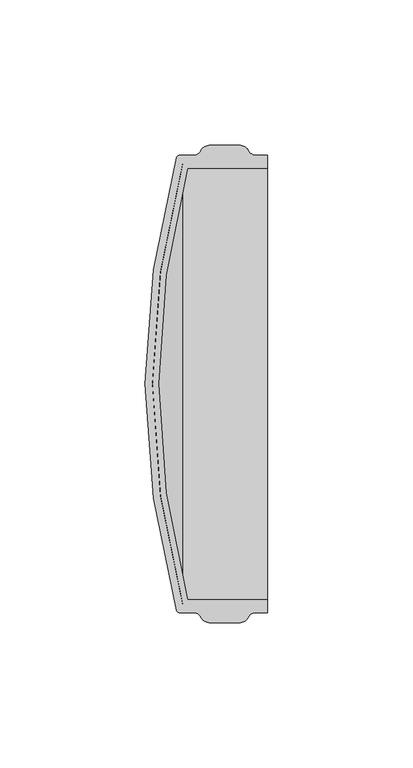
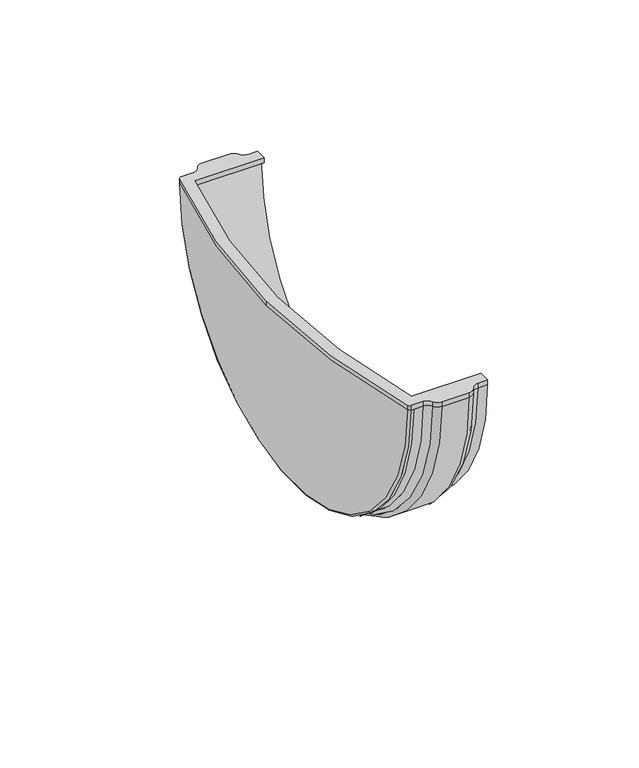
"""IFC4 building model written with IfcOpenShell, lengths in millimetres: proxy geometry, ↩ Заглушка желоба : ↩ Заглушка желоба."""

from ifc_helpers import new_model, si_unit, point, frame, origin, place, context, project, spatial, polyline, circle_curve, ellipse_curve, trimmed, source, transform, mapped, element, save
from ifc_brep_helpers import plane_surface, cylinder_surface, revolved_surface, advanced_brep


def generic_models_4d5a007a(model_context):
    return source(origin(), model_context, "Body", "AdvancedBrep", [
        advanced_brep(
        [(-25.5074023, 78.6, 0.0), (-25.5074023, -78.6, 0.0), (-29.0, -78.6, 0.0), (-29.0, 78.6, 0.0), (-22.8037012, 80.3, 0.0), (-22.8037012, -80.3, 0.0), (-20.1, 82.0, 0.0), (-20.1, -82.0, 0.0), (-9.3443413, 82.0, 0.0), (-9.3443413, -82.0, 0.0), (-6.6406401, 80.3, 0.0), (-6.6406401, -80.3, 0.0), (-3.936939, 78.6, 0.0), (-3.936939, -78.6, 0.0), (-0.0443413, 78.6, 0.0), (-0.0443413, -78.6, 0.0), (-0.0443413, 78.6, 2.0), (-0.0443413, 74.1, 2.0), (-0.0443413, 74.1, 0.0), (-0.0443413, 76.1, 0.0), (-0.0443413, -76.1, 0.0), (-0.0443413, -74.1, 0.0), (-0.0443413, -74.1, 2.0), (-0.0443413, -78.6, 2.0), (-29.0, 76.1, 0.0), (-29.0, -76.1, 0.0), (-31.2572877, 77.8330313, 0.0), (-31.2572877, -77.8330313, 0.0), (-42.0295138, 0.0, 0.0), (-30.2504109, 78.6, 0.0), (-30.2504109, -78.6, 0.0), (-39.5258282, 0.0, 0.0), (-3.936939, 78.6, 2.0), (-6.6406401, 80.3, 2.0), (-9.3443413, 82.0, 2.0), (-20.1, 82.0, 2.0), (-22.8037012, 80.3, 2.0), (-25.5074023, 78.6, 2.0), (-30.2504109, 78.6, 2.0), (-31.2572877, 77.8330313, 2.0), (-42.0295138, 0.0, 2.0), (-31.2572877, -77.8330313, 2.0), (-30.2504109, -78.6, 2.0), (-25.5074023, -78.6, 2.0), (-22.8037012, -80.3, 2.0), (-20.1, -82.0, 2.0), (-9.3443413, -82.0, 2.0), (-6.6406401, -80.3, 2.0), (-3.936939, -78.6, 2.0), (-27.4693868, -74.1, 2.0), (-37.5257643, 0.0, 2.0), (-27.4693868, 74.1, 2.0), (-27.4693868, 74.1, 0.0), (-37.5257643, 0.0, 0.0), (-27.4693868, -74.1, 0.0)],
        [
            (0, 1, circle_curve(frame((-25.5074023, 0.0, 0.0), z_axis=(-1.0, 0.0, 0.0), x_axis=(0.0, -1.0, 0.0)), 78.6)),
            (1, 2),
            (2, 3, circle_curve(frame((-29.0, 0.0, 0.0), z_axis=(1.0, 0.0, 0.0), x_axis=(0.0, -1.0, 0.0)), 78.6)),
            (3, 0),
            (0, 4, circle_curve(frame((-25.5074023, 81.6, 0.0), z_axis=(0.0, 0.0, 1.0), x_axis=(1.0, 0.0, 0.0)), 3.0)),
            (4, 5, circle_curve(frame((-22.8037012, 0.0, 0.0), z_axis=(-1.0, 0.0, 0.0), x_axis=(0.0, -1.0, 0.0)), 80.3)),
            (5, 1, circle_curve(frame((-25.5074023, -81.6, 0.0), z_axis=(0.0, 0.0, 1.0), x_axis=(1.0, 0.0, 0.0)), 3.0)),
            (4, 6, circle_curve(frame((-20.1, 79.0, 0.0), z_axis=(0.0, 0.0, -1.0), x_axis=(1.0, 0.0, 0.0)), 3.0)),
            (6, 7, circle_curve(frame((-20.1, 0.0, 0.0), z_axis=(-1.0, 0.0, 0.0), x_axis=(0.0, -1.0, 0.0)), 82.0)),
            (7, 5, circle_curve(frame((-20.1, -79.0, 0.0), z_axis=(0.0, 0.0, -1.0), x_axis=(1.0, 0.0, 0.0)), 3.0)),
            (6, 8),
            (8, 9, circle_curve(frame((-9.3443413, 0.0, 0.0), z_axis=(-1.0, 0.0, 0.0), x_axis=(0.0, -1.0, 0.0)), 82.0)),
            (9, 7),
            (8, 10, circle_curve(frame((-9.3443413, 79.0, 0.0), z_axis=(0.0, 0.0, -1.0), x_axis=(-1.0, 0.0, 0.0)), 3.0)),
            (10, 11, circle_curve(frame((-6.6406401, 0.0, 0.0), z_axis=(-1.0, 0.0, 0.0), x_axis=(0.0, -1.0, 0.0)), 80.3)),
            (11, 9, circle_curve(frame((-9.3443413, -79.0, 0.0), z_axis=(0.0, 0.0, -1.0), x_axis=(-1.0, 0.0, 0.0)), 3.0)),
            (10, 12, circle_curve(frame((-3.936939, 81.6, 0.0), z_axis=(0.0, 0.0, 1.0), x_axis=(-1.0, 0.0, 0.0)), 3.0)),
            (12, 13, circle_curve(frame((-3.936939, 0.0, 0.0), z_axis=(-1.0, 0.0, 0.0), x_axis=(0.0, -1.0, 0.0)), 78.6)),
            (13, 11, circle_curve(frame((-3.936939, -81.6, 0.0), z_axis=(0.0, 0.0, 1.0), x_axis=(-1.0, 0.0, 0.0)), 3.0)),
            (12, 14),
            (14, 15, circle_curve(frame((-0.0443413, 0.0, 0.0), z_axis=(-1.0, 0.0, 0.0), x_axis=(0.0, -1.0, 0.0)), 78.6)),
            (15, 13),
            (14, 16),
            (16, 17),
            (17, 18),
            (18, 19),
            (19, 20, circle_curve(frame((-0.0443413, 0.0, 0.0), z_axis=(-1.0, 0.0, 0.0), x_axis=(0.0, -1.0, 0.0)), 76.1)),
            (20, 21),
            (21, 22),
            (22, 23),
            (23, 15),
            (19, 24),
            (24, 25, circle_curve(frame((-29.0, 0.0, 0.0), z_axis=(-1.0, 0.0, 0.0), x_axis=(0.0, -1.0, 0.0)), 76.1)),
            (25, 20),
            (26, 27, circle_curve(frame((-31.2572877, 0.0, 0.0), z_axis=(-1.0, 0.0, 0.0), x_axis=(0.0, -1.0, 0.0)), 77.8330313)),
            (27, 28, circle_curve(frame((257.964734, 1.8577595, 0.0), z_axis=(0.0, 0.0, -1.0), x_axis=(1.0, 0.0, 0.0)), 300.0)),
            (28, 26, circle_curve(frame((257.964734, -1.8577595, 0.0), z_axis=(0.0, 0.0, -1.0), x_axis=(1.0, 0.0, 0.0)), 300.0)),
            (26, 29, circle_curve(frame((-30.2504109, 77.5556015, 0.0), z_axis=(0.0, 0.0, -1.0), x_axis=(1.0, 0.0, 0.0)), 1.0443985)),
            (29, 30, circle_curve(frame((-30.2504109, 0.0, 0.0), z_axis=(-1.0, 0.0, 0.0), x_axis=(0.0, -1.0, 0.0)), 78.6)),
            (30, 27, circle_curve(frame((-30.2504109, -77.5556015, 0.0), z_axis=(0.0, 0.0, -1.0), x_axis=(1.0, 0.0, 0.0)), 1.0443985)),
            (29, 3),
            (2, 30),
            (24, 31, circle_curve(frame((257.964734, -2.3696848, 0.0), z_axis=(0.0, 0.0, 1.0), x_axis=(1.0, 0.0, 0.0)), 297.5)),
            (31, 25, circle_curve(frame((257.964734, 2.3696848, 0.0), z_axis=(0.0, 0.0, 1.0), x_axis=(1.0, 0.0, 0.0)), 297.5)),
            (16, 32),
            (32, 33, circle_curve(frame((-3.936939, 81.6, 2.0), z_axis=(0.0, 0.0, -1.0), x_axis=(1.0, 0.0, 0.0)), 3.0)),
            (33, 34, circle_curve(frame((-9.3443413, 79.0, 2.0), z_axis=(0.0, 0.0, 1.0), x_axis=(1.0, 0.0, 0.0)), 3.0)),
            (34, 35),
            (35, 36, circle_curve(frame((-20.1, 79.0, 2.0), z_axis=(0.0, 0.0, 1.0), x_axis=(1.0, 0.0, 0.0)), 3.0)),
            (36, 37, circle_curve(frame((-25.5074023, 81.6, 2.0), z_axis=(0.0, 0.0, -1.0), x_axis=(1.0, 0.0, 0.0)), 3.0)),
            (37, 38),
            (38, 39, circle_curve(frame((-30.2504109, 77.5556015, 2.0), z_axis=(0.0, 0.0, 1.0), x_axis=(1.0, 0.0, 0.0)), 1.0443985)),
            (39, 40, circle_curve(frame((257.964734, -1.8577595, 2.0), z_axis=(0.0, 0.0, 1.0), x_axis=(1.0, 0.0, 0.0)), 300.0)),
            (40, 41, circle_curve(frame((257.964734, 1.8577595, 2.0), z_axis=(0.0, 0.0, 1.0), x_axis=(1.0, 0.0, 0.0)), 300.0)),
            (41, 42, circle_curve(frame((-30.2504109, -77.5556015, 2.0), z_axis=(0.0, 0.0, 1.0), x_axis=(1.0, 0.0, 0.0)), 1.0443985)),
            (42, 43),
            (43, 44, circle_curve(frame((-25.5074023, -81.6, 2.0), z_axis=(0.0, 0.0, -1.0), x_axis=(1.0, 0.0, 0.0)), 3.0)),
            (44, 45, circle_curve(frame((-20.1, -79.0, 2.0), z_axis=(0.0, 0.0, 1.0), x_axis=(1.0, 0.0, 0.0)), 3.0)),
            (45, 46),
            (46, 47, circle_curve(frame((-9.3443413, -79.0, 2.0), z_axis=(0.0, 0.0, 1.0), x_axis=(1.0, 0.0, 0.0)), 3.0)),
            (47, 48, circle_curve(frame((-3.936939, -81.6, 2.0), z_axis=(0.0, 0.0, -1.0), x_axis=(1.0, 0.0, 0.0)), 3.0)),
            (48, 23),
            (22, 49),
            (49, 50, circle_curve(frame((257.964734, 2.3696848, 2.0), z_axis=(0.0, 0.0, -1.0), x_axis=(1.0, 0.0, 0.0)), 295.5)),
            (50, 51, circle_curve(frame((257.964734, -2.3696848, 2.0), z_axis=(0.0, 0.0, -1.0), x_axis=(1.0, 0.0, 0.0)), 295.5)),
            (51, 17),
            (18, 52),
            (52, 53, circle_curve(frame((257.964734, -2.3696848, 0.0), z_axis=(0.0, 0.0, 1.0), x_axis=(1.0, 0.0, 0.0)), 295.5)),
            (53, 54, circle_curve(frame((257.964734, 2.3696848, 0.0), z_axis=(0.0, 0.0, 1.0), x_axis=(1.0, 0.0, 0.0)), 295.5)),
            (54, 21),
            (12, 32),
            (10, 33),
            (8, 34),
            (6, 35),
            (4, 36),
            (0, 37),
            (29, 38),
            (26, 39),
            (28, 40),
            (27, 41),
            (30, 42),
            (1, 43),
            (5, 44),
            (7, 45),
            (9, 46),
            (11, 47),
            (13, 48),
            (54, 49),
            (53, 50),
            (52, 51),
        ],
        [
            cylinder_surface(frame((-14.7221706, 0.0, 0.0), z_axis=(1.0, 0.0, 0.0), x_axis=(0.0, -1.0, 0.0)), 78.6),
            revolved_surface(trimmed(ellipse_curve(frame((-25.5074023, -81.6, 0.0), z_axis=(0.0, 0.0, -1.0), x_axis=(1.0, 0.0, 0.0)), 3.0, 3.0), [point((-25.5074023, -78.6, 0.0))], [point((-22.8037012, -80.3, 0.0))], True, "CARTESIAN"), (-14.7221706, 0.0, 0.0), (1.0, 0.0, 0.0)),
            revolved_surface(trimmed(ellipse_curve(frame((-20.1, -79.0, 0.0), z_axis=(0.0, 0.0, 1.0), x_axis=(1.0, 0.0, 0.0)), 3.0, 3.0), [point((-22.8037012, -80.3, 0.0))], [point((-20.1, -82.0, 0.0))], True, "CARTESIAN"), (-14.7221706, 0.0, 0.0), (1.0, 0.0, 0.0)),
            cylinder_surface(frame((-14.7221706, 0.0, 0.0), z_axis=(1.0, 0.0, 0.0), x_axis=(0.0, -1.0, 0.0)), 82.0),
            revolved_surface(trimmed(ellipse_curve(frame((-9.3443413, -79.0, 0.0), z_axis=(0.0, 0.0, 1.0), x_axis=(-1.0, 0.0, 0.0)), 3.0, 3.0), [point((-9.3443413, -82.0, 0.0))], [point((-6.6406401, -80.3, 0.0))], True, "CARTESIAN"), (-14.7221706, 0.0, 0.0), (1.0, 0.0, 0.0)),
            revolved_surface(trimmed(ellipse_curve(frame((-3.936939, -81.6, 0.0), z_axis=(0.0, 0.0, -1.0), x_axis=(-1.0, 0.0, 0.0)), 3.0, 3.0), [point((-6.6406401, -80.3, 0.0))], [point((-3.936939, -78.6, 0.0))], True, "CARTESIAN"), (-14.7221706, 0.0, 0.0), (1.0, 0.0, 0.0)),
            plane_surface(frame((-0.0443413, 0.0, 0.0), z_axis=(1.0, 0.0, 0.0), x_axis=(0.0, -1.0, 0.0))),
            revolved_surface(polyline([(-0.04434129999999925, -76.1, 0.0), (-29.0, -76.1, 0.0)]), (-14.7221706, 0.0, 0.0), (1.0, 0.0, 0.0)),
            revolved_surface(trimmed(ellipse_curve(frame((257.964734, 1.8577595, 0.0), z_axis=(0.0, 0.0, 1.0), x_axis=(1.0, 0.0, 0.0)), 300.0, 300.0), [point((-42.0295138, 0.0, 0.0))], [point((-31.2572877, -77.8330313, 0.0))], True, "CARTESIAN"), (-42.0, 0.0, 0.0), (1.0, 0.0, 0.0)),
            revolved_surface(trimmed(ellipse_curve(frame((-30.2504109, -77.5556015, 0.0), z_axis=(0.0, 0.0, 1.0), x_axis=(1.0, 0.0, 0.0)), 1.0443985, 1.0443985), [point((-31.2572877, -77.8330313, 0.0))], [point((-30.2504109, -78.6, 0.0))], True, "CARTESIAN"), (-42.0, 0.0, 0.0), (1.0, 0.0, 0.0)),
            cylinder_surface(frame((-42.0, 0.0, 0.0), z_axis=(1.0, 0.0, 0.0), x_axis=(0.0, -1.0, 0.0)), 78.6),
            revolved_surface(trimmed(ellipse_curve(frame((257.964734, 2.3696848, 0.0), z_axis=(0.0, 0.0, -1.0), x_axis=(1.0, 0.0, 0.0)), 297.5, 297.5), [point((-29.0, -76.1, 0.0))], [point((-39.5258282, 0.0, 0.0))], True, "CARTESIAN"), (-42.0, 0.0, 0.0), (1.0, 0.0, 0.0)),
            plane_surface(frame((-0.0443413, 78.6, 2.0), z_axis=(0.0, 0.0, 1.0), x_axis=(-1.0, 0.0, 0.0))),
            plane_surface(frame((-0.0443413, 78.6, 0.0), z_axis=(0.0, 0.0, -1.0), x_axis=(1.0, 0.0, 0.0))),
            plane_surface(frame((-0.0443413, 78.6, 2.0), z_axis=(0.0, 1.0, 0.0), x_axis=(0.0, 0.0, -1.0))),
            revolved_surface(polyline([(-0.9369390000000002, 81.6, 0.0), (-0.9369390000000002, 81.6, 2.0)]), (-3.936939, 81.6, 0.0), (0.0, 0.0, -1.0)),
            cylinder_surface(frame((-9.3443413, 79.0, 0.0), z_axis=(0.0, 0.0, 1.0), x_axis=(1.0, 0.0, 0.0)), 3.0),
            plane_surface(frame((-9.3443413, 82.0, 2.0), z_axis=(0.0, 1.0, 0.0), x_axis=(0.0, 0.0, -1.0))),
            cylinder_surface(frame((-20.1, 79.0, 0.0), z_axis=(0.0, 0.0, 1.0), x_axis=(1.0, 0.0, 0.0)), 3.0),
            revolved_surface(polyline([(-22.5074023, 81.6, 0.0), (-22.5074023, 81.6, 2.0)]), (-25.5074023, 81.6, 0.0), (0.0, 0.0, -1.0)),
            plane_surface(frame((-25.5074023, 78.6, 2.0), z_axis=(0.0, 1.0, 0.0), x_axis=(0.0, 0.0, -1.0))),
            cylinder_surface(frame((-30.2504109, 77.5556015, 0.0), z_axis=(0.0, 0.0, 1.0), x_axis=(1.0, 0.0, 0.0)), 1.0443985),
            cylinder_surface(frame((257.964734, -1.8577595, 0.0), z_axis=(0.0, 0.0, 1.0), x_axis=(1.0, 0.0, 0.0)), 300.0),
            cylinder_surface(frame((257.964734, 1.8577595, 0.0), z_axis=(0.0, 0.0, 1.0), x_axis=(1.0, 0.0, 0.0)), 300.0),
            cylinder_surface(frame((-30.2504109, -77.5556015, 0.0), z_axis=(0.0, 0.0, 1.0), x_axis=(1.0, 0.0, 0.0)), 1.0443985),
            plane_surface(frame((-30.2504109, -78.6, 2.0), z_axis=(0.0, -1.0, 0.0), x_axis=(0.0, 0.0, -1.0))),
            revolved_surface(polyline([(-22.5074023, -81.6, 0.0), (-22.5074023, -81.6, 2.0)]), (-25.5074023, -81.6, 0.0), (0.0, 0.0, -1.0)),
            cylinder_surface(frame((-20.1, -79.0, 0.0), z_axis=(0.0, 0.0, 1.0), x_axis=(1.0, 0.0, 0.0)), 3.0),
            plane_surface(frame((-20.1, -82.0, 2.0), z_axis=(0.0, -1.0, 0.0), x_axis=(0.0, 0.0, -1.0))),
            cylinder_surface(frame((-9.3443413, -79.0, 0.0), z_axis=(0.0, 0.0, 1.0), x_axis=(1.0, 0.0, 0.0)), 3.0),
            revolved_surface(polyline([(-0.9369390000000002, -81.6, 0.0), (-0.9369390000000002, -81.6, 2.0)]), (-3.936939, -81.6, 0.0), (0.0, 0.0, -1.0)),
            plane_surface(frame((-3.936939, -78.6, 2.0), z_axis=(0.0, -1.0, 0.0), x_axis=(0.0, 0.0, -1.0))),
            plane_surface(frame((-0.0443413, -74.1, 2.0), z_axis=(0.0, 1.0, 0.0), x_axis=(0.0, 0.0, -1.0))),
            revolved_surface(polyline([(553.464734, 2.3696848, 0.0), (553.464734, 2.3696848, 2.0)]), (257.964734, 2.3696848, 0.0), (0.0, 0.0, -1.0)),
            revolved_surface(polyline([(553.464734, -2.3696848, 0.0), (553.464734, -2.3696848, 2.0)]), (257.964734, -2.3696848, 0.0), (0.0, 0.0, -1.0)),
            plane_surface(frame((-27.4693868, 74.1, 2.0), z_axis=(0.0, -1.0, 0.0), x_axis=(0.0, 0.0, -1.0))),
        ],
        [
            (0, [[1, 2, 3, 4]]),
            (1, [[-1, 5, 6, 7]]),
            (2, [[-6, 8, 9, 10]]),
            (3, [[-9, 11, 12, 13]]),
            (4, [[-12, 14, 15, 16]]),
            (5, [[-15, 17, 18, 19]]),
            (0, [[-18, 20, 21, 22]]),
            (6, [[-21, 23, 24, 25, 26, 27, 28, 29, 30, 31]]),
            (7, [[-27, 32, 33, 34]]),
            (8, [[35, 36, 37]]),
            (9, [[-35, 38, 39, 40]]),
            (10, [[-39, 41, -3, 42]]),
            (11, [[-33, 43, 44]]),
            (12, [[45, 46, 47, 48, 49, 50, 51, 52, 53, 54, 55, 56, 57, 58, 59, 60, 61, 62, -30, 63, 64, 65, 66, -24]]),
            (13, [[67, 68, 69, 70, -28, -34, -44, -43, -32, -26]]),
            (14, [[-45, -23, -20, 71]]),
            (15, [[-46, -71, -17, 72]]),
            (16, [[-47, -72, -14, 73]]),
            (17, [[-48, -73, -11, 74]]),
            (18, [[-49, -74, -8, 75]]),
            (19, [[-50, -75, -5, 76]]),
            (20, [[-51, -76, -4, -41, 77]]),
            (21, [[-52, -77, -38, 78]]),
            (22, [[-53, -78, -37, 79]]),
            (23, [[-54, -79, -36, 80]]),
            (24, [[-55, -80, -40, 81]]),
            (25, [[-56, -81, -42, -2, 82]]),
            (26, [[-57, -82, -7, 83]]),
            (27, [[-58, -83, -10, 84]]),
            (28, [[-59, -84, -13, 85]]),
            (29, [[-60, -85, -16, 86]]),
            (30, [[-61, -86, -19, 87]]),
            (31, [[-62, -87, -22, -31]]),
            (32, [[-63, -29, -70, 88]]),
            (33, [[-64, -88, -69, 89]]),
            (34, [[-65, -89, -68, 90]]),
            (35, [[-66, -90, -67, -25]]),
        ],
    ),
    ])


if __name__ == "__main__":
    model = new_model("IFC4")
    model_context = context("Model", 3, world=origin())
    ifc_project = project(units=[si_unit("LENGTHUNIT", "METRE", prefix="MILLI")], contexts=[model_context])
    site = spatial("IfcSite", under=ifc_project)
    building = spatial("IfcBuilding", under=site)
    placement = place(None, origin())
    generic_models_shape = generic_models_4d5a007a(model_context)
    element("IfcBuildingElementProxy", 1, Name="↩ Заглушка желоба : ↩ Заглушка желоба", ObjectType="↩ Заглушка желоба : ↩ Заглушка желоба", at=placement, inside=building, context=model_context, shape_type="MappedRepresentation", body=[
        mapped(generic_models_shape, transform((0.0, 0.0, 0.0), x_axis=(1.0, 0.0, 0.0), y_axis=(0.0, 1.0, 0.0), z_axis=(0.0, 0.0, 1.0))),
    ])
    save(model, "model.ifc")

# Revit data of these elements
# Type "↩ Заглушка желоба : ↩ Заглушка желоба"
#   Description = "Устанавливается на торцах желоба\r\nи направляет дождевую воду в сторону\r\nуклона к воронке."
#   Manufacturer = "ТехноНИКОЛЬ"
#   Model = "Комплектующие к водосточным системам"
#   URL = "https://tn-vodostok.ru/catalog/pvh/"
#   ADSK_Обозначение = "ТехноНИКОЛЬ"
#   ADSK_Наименование краткое = "Заглушка"
#   ADSK_Наименование = "Заглушка желоба"
#   ADSK_Масса_Текст = ""
#   ADSK_Марка = ""
#   ADSK_Код изделия = ""
#   ADSK_Завод-изготовитель = "ТехноНИКОЛЬ"
#   ADSK_Единица измерения = "шт."
#   ADSK_Группирование = "Комплектующие к водосточным системам"
#   ADSK_URL страницы изделия = "https://tn-vodostok.ru/catalog/pvh/"
#   ADSK_URL документации изделия = "https://tn-vodostok.ru/upload/iblock/c42/c427963cb77eb5c3c51f0cfb870e9e52.pdf"
#   Угол поворота кронштейна [instance default] = 0.00°
#   Длина пластины [instance default] = 0 mm
#   ADSK_Размер_Ширина = 164 mm
#   ADSK_Размер_Длина = 42 mm
#   ADSK_Размер_Высота = 82 mm
#   ADSK_Количество = 1
#   Видимость_Защитная решетка [instance default] = yes
#   Материал_Защитная решетка [instance default] = none
#   ADSK_Материал [instance default] = TN_Пластик_Коричневый_RAL8019
#   Default Elevation = 0
# Element 1 (IfcBuildingElementProxy, "↩ Заглушка желоба : ↩ Заглушка желоба")
#   Длина пластины = 200 mm
#   Материал_Защитная решетка = TN_Пластик_Решетка_Коричневый_RAL8019
#   Materials on its faces: "TN_Пластик_Коричневый_RAL8019"
# Materials
#   "TN_Пластик_Коричневый_RAL8019": class "Типовые", colour RGB 61 54 53, transparency 0, Cost = 0
#   "TN_Пластик_Решетка_Коричневый_RAL8019": class "Типовые", colour RGB 61 54 53, transparency 0.25, Cost = 0
